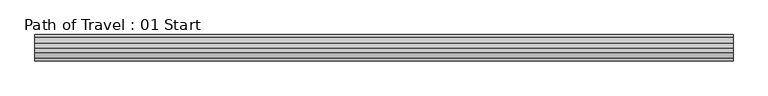
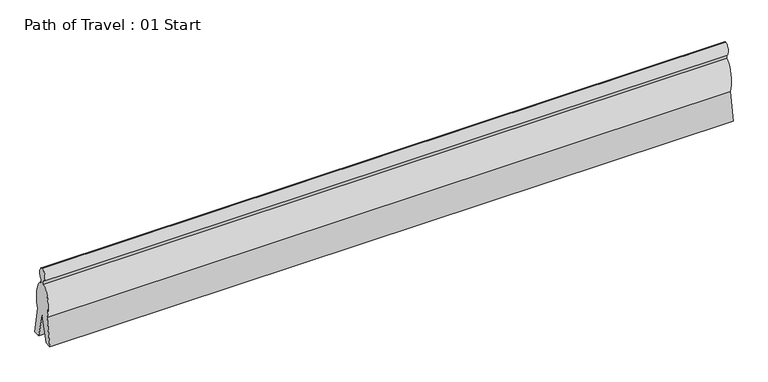
"""IFC4 building model written with IfcOpenShell, lengths in millimetres: proxy geometry, Path of Travel : 01 Start."""

from ifc_helpers import new_model, si_unit, point, frame, origin, place, context, project, spatial, ellipse_curve, trimmed, source, transform, mapped, element, save
from ifc_brep_helpers import plane_surface, extruded_surface, advanced_brep


def path_of_travel_01_start_5b2d4024(model_context):
    return source(origin(), model_context, "Body", "AdvancedBrep", [
        advanced_brep(
        [(227.5554837, 0.0, 1727.2), (227.5554837, 42.9018657, 1436.6534209), (227.5554837, 42.9018657, 1363.4763406), (227.5554837, 184.1186263, 643.4144547), (227.5554837, 297.5699544, 0.0), (227.5554837, 145.6574193, 0.0), (227.5554837, 0.0, 584.2), (227.5554837, -145.6574193, 0.0), (227.5554837, -297.5699544, 0.0), (227.5554837, -184.1186263, 643.4144547), (227.5554837, -42.9018657, 1363.4763406), (227.5554837, -42.9018657, 1436.6534209), (15899.3554837, 0.0, 1727.2), (15899.3554837, -42.9018657, 1436.6534209), (15899.3554837, -42.9018657, 1363.4763406), (15899.3554837, -184.1186263, 643.4144547), (15899.3554837, -297.5699544, 0.0), (15899.3554837, -145.6574193, 0.0), (15899.3554837, 0.0, 584.2), (15899.3554837, 145.6574193, 0.0), (15899.3554837, 297.5699544, 0.0), (15899.3554837, 184.1186263, 643.4144547), (15899.3554837, 42.9018657, 1363.4763406), (15899.3554837, 42.9018657, 1436.6534209)],
        [
            (0, 1, ellipse_curve(frame((227.5554837, 0.0, 1574.8), z_axis=(-1.0, 0.0, 0.0), x_axis=(0.0, 0.0, 1.0)), 152.4, 101.6)),
            (1, 2),
            (2, 3, ellipse_curve(frame((227.5554837, 0.0, 914.4), z_axis=(-1.0, 0.0, 0.0), x_axis=(0.0, 0.0, -1.0)), 457.2, 228.6)),
            (3, 4),
            (4, 5),
            (5, 6),
            (6, 7),
            (7, 8),
            (8, 9),
            (9, 10, ellipse_curve(frame((227.5554837, 0.0, 914.4), z_axis=(-1.0, 0.0, 0.0), x_axis=(0.0, 0.0, -1.0)), 457.2, 228.6)),
            (10, 11),
            (11, 0, ellipse_curve(frame((227.5554837, 0.0, 1574.8), z_axis=(-1.0, 0.0, 0.0), x_axis=(0.0, 0.0, 1.0)), 152.4, 101.6)),
            (12, 13, ellipse_curve(frame((15899.3554837, 0.0, 1574.8), z_axis=(1.0, 0.0, 0.0), x_axis=(0.0, 0.0, 1.0)), 152.4, 101.6)),
            (13, 14),
            (14, 15, ellipse_curve(frame((15899.3554837, 0.0, 914.4), z_axis=(1.0, 0.0, 0.0), x_axis=(0.0, 0.0, -1.0)), 457.2, 228.6)),
            (15, 16),
            (16, 17),
            (17, 18),
            (18, 19),
            (19, 20),
            (20, 21),
            (21, 22, ellipse_curve(frame((15899.3554837, 0.0, 914.4), z_axis=(1.0, 0.0, 0.0), x_axis=(0.0, 0.0, -1.0)), 457.2, 228.6)),
            (22, 23),
            (23, 12, ellipse_curve(frame((15899.3554837, 0.0, 1574.8), z_axis=(1.0, 0.0, 0.0), x_axis=(0.0, 0.0, 1.0)), 152.4, 101.6)),
            (11, 13),
            (12, 0),
            (10, 14),
            (9, 15),
            (8, 16),
            (7, 17),
            (6, 18),
            (5, 19),
            (4, 20),
            (3, 21),
            (2, 22),
            (1, 23),
        ],
        [
            plane_surface(frame((227.5554837, 0.0, 0.0), z_axis=(-1.0, 0.0, 0.0), x_axis=(0.0, 0.0, 1.0))),
            plane_surface(frame((15899.3554837, 0.0, 0.0), z_axis=(1.0, 0.0, 0.0), x_axis=(0.0, 0.0, 1.0))),
            extruded_surface(trimmed(ellipse_curve(frame((227.5554837, 0.0, 1574.8), z_axis=(1.0, 0.0, 0.0), x_axis=(0.0, 0.0, 1.0)), 152.4, 101.6), [point((227.5554837, 0.0, 1727.2))], [point((227.5554837, -42.9018657, 1436.6534209))], True, "CARTESIAN"), (15671.8, 0.0, 0.0), 15671.8),
            plane_surface(frame((227.5554837, -42.9018657, 1436.6534209), z_axis=(0.0, -1.0, 0.0), x_axis=(1.0, 0.0, 0.0))),
            extruded_surface(trimmed(ellipse_curve(frame((227.5554837, 0.0, 914.4), z_axis=(1.0, 0.0, 0.0), x_axis=(0.0, 0.0, -1.0)), 457.2, 228.6), [point((227.5554837, -42.9018657, 1363.4763406))], [point((227.5554837, -184.1186263, 643.4144547))], True, "CARTESIAN"), (15671.8, 0.0, 0.0), 15671.8),
            plane_surface(frame((227.5554837, -184.1186263, 643.4144547), z_axis=(0.0, -0.9848077530122078, 0.17364817766693205), x_axis=(1.0, 0.0, 0.0))),
            plane_surface(frame((227.5554837, -297.5699544, 0.0), z_axis=(0.0, 0.0, -1.0), x_axis=(1.0, 0.0, 0.0))),
            plane_surface(frame((227.5554837, -145.6574193, 0.0), z_axis=(0.0, 0.9702957262760199, -0.2419218955995739), x_axis=(1.0, 0.0, 0.0))),
            plane_surface(frame((227.5554837, 0.0, 584.2), z_axis=(0.0, -0.9702957262759961, -0.24192189559966923), x_axis=(1.0, 0.0, 0.0))),
            plane_surface(frame((227.5554837, 145.6574193, 0.0), z_axis=(0.0, 0.0, -1.0), x_axis=(1.0, 0.0, 0.0))),
            plane_surface(frame((227.5554837, 297.5699544, 0.0), z_axis=(0.0, 0.984807753012208, 0.17364817766693066), x_axis=(1.0, 0.0, 0.0))),
            extruded_surface(trimmed(ellipse_curve(frame((227.5554837, 0.0, 914.4), z_axis=(1.0, 0.0, 0.0), x_axis=(0.0, 0.0, -1.0)), 457.2, 228.6), [point((227.5554837, 184.1186263, 643.4144547))], [point((227.5554837, 42.9018657, 1363.4763406))], True, "CARTESIAN"), (15671.8, 0.0, 0.0), 15671.8),
            plane_surface(frame((227.5554837, 42.9018657, 1363.4763406), z_axis=(0.0, 1.0, 0.0), x_axis=(1.0, 0.0, 0.0))),
            extruded_surface(trimmed(ellipse_curve(frame((227.5554837, 0.0, 1574.8), z_axis=(1.0, 0.0, 0.0), x_axis=(0.0, 0.0, 1.0)), 152.4, 101.6), [point((227.5554837, 42.9018657, 1436.6534209))], [point((227.5554837, 0.0, 1727.2))], True, "CARTESIAN"), (15671.8, 0.0, 0.0), 15671.8),
        ],
        [
            (0, [[1, 2, 3, 4, 5, 6, 7, 8, 9, 10, 11, 12]]),
            (1, [[13, 14, 15, 16, 17, 18, 19, 20, 21, 22, 23, 24]]),
            (2, [[25, -13, 26, -12]]),
            (3, [[27, -14, -25, -11]]),
            (4, [[28, -15, -27, -10]]),
            (5, [[29, -16, -28, -9]]),
            (6, [[30, -17, -29, -8]]),
            (7, [[31, -18, -30, -7]]),
            (8, [[32, -19, -31, -6]]),
            (9, [[33, -20, -32, -5]]),
            (10, [[34, -21, -33, -4]]),
            (11, [[35, -22, -34, -3]]),
            (12, [[36, -23, -35, -2]]),
            (13, [[-26, -24, -36, -1]]),
        ],
    ),
    ])


if __name__ == "__main__":
    model = new_model("IFC4")
    model_context = context("Model", 3, world=origin())
    ifc_project = project(units=[si_unit("LENGTHUNIT", "METRE", prefix="MILLI")], contexts=[model_context])
    site = spatial("IfcSite", under=ifc_project)
    building = spatial("IfcBuilding", under=site)
    placement = place(None, origin())
    path_of_travel_01_start_shape = path_of_travel_01_start_5b2d4024(model_context)
    element("IfcBuildingElementProxy", 1, Name="Path of Travel : 01 Start", ObjectType="Path of Travel : 01 Start", at=placement, inside=building, context=model_context, shape_type="MappedRepresentation", body=[
        mapped(path_of_travel_01_start_shape, transform((0.0, 0.0, 0.0), x_axis=(1.0, 0.0, 0.0), y_axis=(0.0, 1.0, 0.0), z_axis=(0.0, 0.0, 1.0))),
    ])
    save(model, "model.ifc")

# Revit data of these elements
# Type "Path of Travel : 01 Start"
#   Path of Egress [instance default] = 4' - 0"
#   built-in parameter 1001306 [instance default] = 4 (stored number, unit not read)
#   Dot at Start = yes
#   Arrow in Middle = yes
#   Arrow at End = no
#   Egress Path = none
# Element 1 (IfcBuildingElementProxy, "Path of Travel : 01 Start")
#   Path of Egress = 51' - 5"
#   built-in parameter 1001306 = 51.4167 (stored number, unit not read)
#   Materials on its faces: "Egress Path Solid"
# Materials
#   "Egress Path Solid": class "Unassigned", colour RGB 255 128 64, transparency 0.75, Comments = "Rendering appearance not upgraded "
